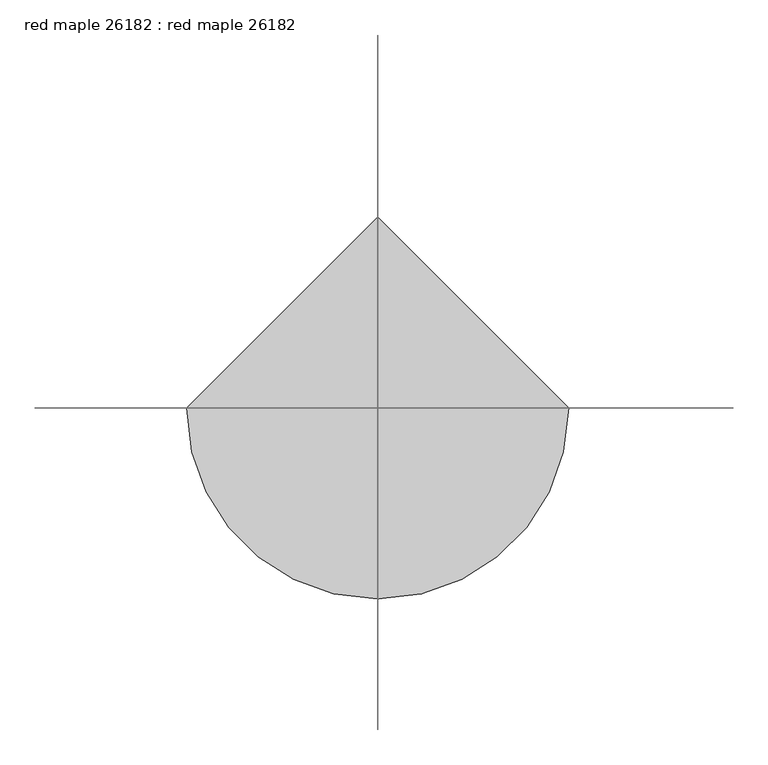
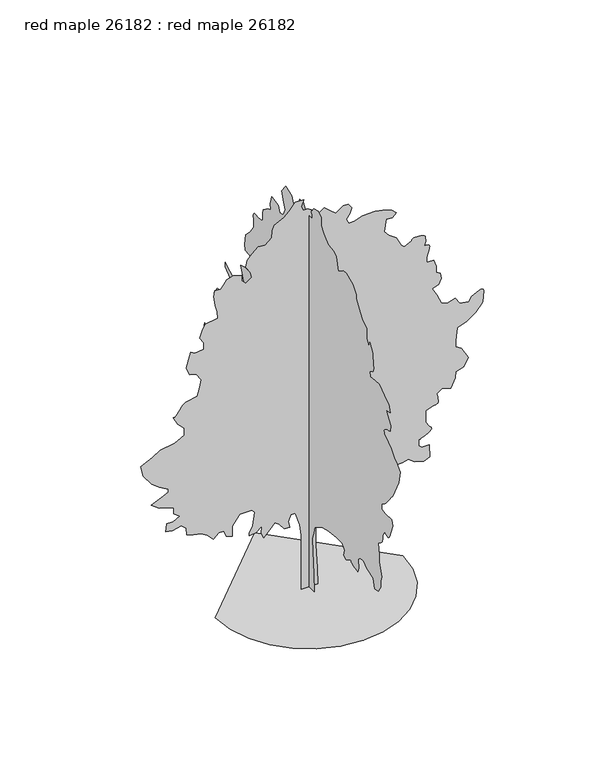
"""IFC4 building model written with IfcOpenShell, lengths in millimetres: proxy geometry, red maple 26182 : red maple 26182."""

import ifcopenshell
import ifcopenshell.guid

model = None  # the IFC model being written
_history = None  # IfcOwnerHistory: only IFC2X3 demands one
_inside = {}  # id of a spatial element -> (the spatial element, [elements in it])
_under = {}  # id of a project, library or spatial element -> (it, [spatial elements below it])
_declared = {}  # id of a project -> (the project, [libraries it declares])
_typed = {}  # id of a type object -> (the type object, [elements of that type])
_made_of = {}  # id of a material, layer set ... -> (it, [elements and type objects made of it])


def new_model(schema):
    """Start an empty IFC model of exactly this schema.

    Asked for "IFC4X3", IfcOpenShell would pick the latest addendum, in which some entities
    have other attributes; the version numbers below select the first issue.
    IFC2X3 requires an IfcOwnerHistory on every rooted entity: one is made here for all.
    """
    global model, _history
    if schema == "IFC4X3":
        model = ifcopenshell.file(schema_version=(4, 3, 0, 0))
    else:
        model = ifcopenshell.file(schema=schema)
    _inside.clear()
    _under.clear()
    _declared.clear()
    _typed.clear()
    _made_of.clear()
    _history = None
    if model.schema == "IFC2X3":
        org = make("IfcOrganization", Name="unknown")
        user = make(
            "IfcPersonAndOrganization",
            ThePerson=make("IfcPerson", FamilyName="unknown"),
            TheOrganization=org,
        )
        app = make(
            "IfcApplication",
            ApplicationDeveloper=org,
            Version="unknown",
            ApplicationFullName="unknown",
            ApplicationIdentifier="unknown",
        )
        _history = make(
            "IfcOwnerHistory",
            OwningUser=user,
            OwningApplication=app,
            ChangeAction="ADDED",
            CreationDate=0,
        )
    return model


def make(cls, **values):
    """One entity of the class cls with the attributes given. An attribute that is None is left unset."""
    return model.create_entity(
        cls, **{name: value for name, value in values.items() if value is not None}
    )


def rooted(cls, **values):
    """An entity with a GlobalId (a new one), such as an element, a storey or a relation."""
    return make(cls, GlobalId=ifcopenshell.guid.new(), OwnerHistory=_history, **values)


def si_unit(unit_type, name, prefix=None):
    """IfcSIUnit, for example si_unit("LENGTHUNIT", "METRE", prefix="MILLI")."""
    return make("IfcSIUnit", UnitType=unit_type, Prefix=prefix, Name=name)


def assignment(units):
    """IfcUnitAssignment: the units of a project."""
    return None if units is None else make("IfcUnitAssignment", Units=units)


def point(xyz):
    """IfcCartesianPoint."""
    return None if xyz is None else make("IfcCartesianPoint", Coordinates=xyz)


def direction(xyz):
    """IfcDirection."""
    return None if xyz is None else make("IfcDirection", DirectionRatios=xyz)


def frame(location, z_axis=None, x_axis=None):
    """IfcAxis2Placement3D, a coordinate frame: its origin and axes. An axis left out is left unset."""
    return make(
        "IfcAxis2Placement3D",
        Location=point(location),
        Axis=direction(z_axis),
        RefDirection=direction(x_axis),
    )


def origin():
    """The frame at (0, 0, 0) with its axes left unset."""
    return frame((0.0, 0.0, 0.0))


def place(relative_to, where):
    """IfcLocalPlacement: puts the frame where relative to a parent placement (None: the world)."""
    return make(
        "IfcLocalPlacement", PlacementRelTo=relative_to, RelativePlacement=where
    )


def context(
    kind, dimensions, precision=None, world=None, true_north=None, identifier=None
):
    """IfcGeometricRepresentationContext, for example the 3D "Model" context."""
    return make(
        "IfcGeometricRepresentationContext",
        ContextIdentifier=identifier,
        ContextType=kind,
        CoordinateSpaceDimension=dimensions,
        Precision=precision,
        WorldCoordinateSystem=world,
        TrueNorth=true_north,
    )


def project(units=None, contexts=None):
    """IfcProject with its units and contexts."""
    return rooted(
        "IfcProject",
        Name="project",
        RepresentationContexts=contexts,
        UnitsInContext=assignment(units),
    )


def spatial(cls, under=None, at=None, **own):
    """A site, building, storey or space (cls), placed at a placement, below another one or the project."""
    s = rooted(cls, ObjectPlacement=at, **own)
    if under is not None:
        _under.setdefault(under.id(), (under, []))[1].append(s)
    return s


def point_list(points):
    """IfcCartesianPointList2D or 3D."""
    cls = (
        "IfcCartesianPointList2D" if len(points[0]) == 2 else "IfcCartesianPointList3D"
    )
    return make(cls, CoordList=points)


def triangles(points, corners, closed=None, point_numbers=None):
    """IfcTriangulatedFaceSet: each triangle names its three corners, points numbered from 1."""
    return make(
        "IfcTriangulatedFaceSet",
        Coordinates=point_list(points),
        Closed=closed,
        CoordIndex=corners,
        PnIndex=point_numbers,
    )


def shape(context_of_items, identifier, shape_type, items):
    """IfcShapeRepresentation: the items that make up one representation, for example the "Body"."""
    return make(
        "IfcShapeRepresentation",
        ContextOfItems=context_of_items,
        RepresentationIdentifier=identifier,
        RepresentationType=shape_type,
        Items=items,
    )


def source(mapping_origin, context_of_items, identifier, shape_type, items):
    """IfcRepresentationMap: a shape defined once, which mapped items show again and again."""
    return make(
        "IfcRepresentationMap",
        MappingOrigin=mapping_origin,
        MappedRepresentation=shape(context_of_items, identifier, shape_type, items),
    )


def transform(
    local_origin,
    x_axis=None,
    y_axis=None,
    z_axis=None,
    scale=None,
    scale2=None,
    scale3=None,
    uniform=True,
):
    """IfcCartesianTransformationOperator3D, or its non-uniform kind. x_axis, y_axis, z_axis: its Axis1, 2, 3."""
    if uniform:
        return make(
            "IfcCartesianTransformationOperator3D",
            Axis1=direction(x_axis),
            Axis2=direction(y_axis),
            LocalOrigin=point(local_origin),
            Scale=scale,
            Axis3=direction(z_axis),
        )
    return make(
        "IfcCartesianTransformationOperator3DnonUniform",
        Axis1=direction(x_axis),
        Axis2=direction(y_axis),
        LocalOrigin=point(local_origin),
        Scale=scale,
        Axis3=direction(z_axis),
        Scale2=scale2,
        Scale3=scale3,
    )


def mapped(mapping_source, mapping_target):
    """IfcMappedItem: shows the shape of a source again, moved by a transform."""
    return make(
        "IfcMappedItem", MappingSource=mapping_source, MappingTarget=mapping_target
    )


def made_of(thing, what):
    """Note that an element or type object is made of a material, layer set ...; save() writes the relation."""
    if what is not None:
        _made_of.setdefault(what.id(), (what, []))[1].append(thing)
    return thing


def element(
    cls,
    number,
    at=None,
    inside=None,
    cuts=None,
    type_object=None,
    material=None,
    context=None,
    identifier="Body",
    shape_type=None,
    held_by="IfcProductDefinitionShape",
    body=None,
    shapes=None,
    **own,
):
    """One element of the class cls, such as IfcWall. Its Tag is "e" and its number.

    at: its placement. inside: the storey or other place that contains it. cuts: it is an
    opening in that element (IfcRelVoidsElement). A single representation is given by context,
    identifier, shape_type and body (its items); several are given by shapes. held_by: the class
    of the entity that holds the representations. save() writes the other relations.
    """
    e = rooted(cls, Tag="e%d" % number, ObjectPlacement=at, **own)
    if body is not None:
        shapes = [shape(context, identifier, shape_type, body)]
    if shapes is not None:
        e.Representation = make(held_by, Representations=shapes)
    if inside is not None:
        _inside.setdefault(inside.id(), (inside, []))[1].append(e)
    if cuts is not None:
        rooted(
            "IfcRelVoidsElement", RelatingBuildingElement=cuts, RelatedOpeningElement=e
        )
    if type_object is not None:
        _typed.setdefault(type_object.id(), (type_object, []))[1].append(e)
    return made_of(e, material)


def aggregate(whole, parts):
    """IfcRelAggregates: a whole, such as a stair, and the parts it consists of."""
    return rooted("IfcRelAggregates", RelatingObject=whole, RelatedObjects=parts)


def save(model, path):
    """Write the relations noted so far, then the file.

    IfcRelAggregates (storeys below a building ...), IfcRelContainedInSpatialStructure (elements
    in a storey), IfcRelDefinesByType, IfcRelAssociatesMaterial and IfcRelDeclares: one each for
    every whole, place, type object, material and project.
    """
    for whole, parts in _under.values():
        aggregate(whole, parts)
    for where, things in _inside.values():
        rooted(
            "IfcRelContainedInSpatialStructure",
            RelatedElements=things,
            RelatingStructure=where,
        )
    for kind, things in _typed.values():
        rooted("IfcRelDefinesByType", RelatedObjects=things, RelatingType=kind)
    for what, things in _made_of.values():
        rooted("IfcRelAssociatesMaterial", RelatedObjects=things, RelatingMaterial=what)
    for by, libraries in _declared.values():
        rooted("IfcRelDeclares", RelatingContext=by, RelatedDefinitions=libraries)
    model.write(path)


def red_maple_26182_red_maple_26182_cba750cc(model_context):
    return source(origin(), model_context, "Body", "Tessellation", [
        triangles([(5.9e-06, 200.5240248, 0.0131599), (5.9e-06, -200.5423013, 0.0131599), (5.9e-06, -173.8047255, 401.079007), (5.9e-06, -147.0663684, 922.4677488), (5.9e-06, -133.6980892, 1216.5822092), (5.9e-06, -173.8047255, 1363.6407475), (5.9e-06, -227.2806583, 1537.4352264), (5.9e-06, -320.8632274, 1590.9124855), (5.9e-06, -534.7644153, 1711.2323215), (5.9e-06, -762.0361897, 1764.7071098), (5.9e-06, -1069.5212002, 1804.8136734), (5.9e-06, -1283.4223881, 1804.8136734), (5.9e-06, -1377.0037399, 1697.8617714), (5.9e-06, -1336.897031, 1550.8033058), (5.9e-06, -1443.848933, 1510.6967422), (5.9e-06, -1617.6460281, 1604.2805649), (5.9e-06, -1620.762553, 1592.8200726), (5.9e-06, -1625.400642, 1581.362051), (5.9e-06, -1633.0790977, 1569.9041748), (5.9e-06, -1645.319339, 1558.4436825), (5.9e-06, -1663.6378429, 1546.9856609), (5.9e-06, -1689.5560284, 1535.5251686), (5.9e-06, -1724.595314, 1524.0672924), (5.9e-06, -1761.1942429, 1514.1662979), (5.9e-06, -1791.4812023, 1507.0721088), (5.9e-06, -1816.5027855, 1502.3197826), (5.9e-06, -1837.3156139, 1499.4343483), (5.9e-06, -1854.971077, 1497.9534794), (5.9e-06, -1870.5234707, 1497.4074371), (5.9e-06, -1885.021859, 1497.3286629), (5.9e-06, -1911.7604885, 1590.9124855), (5.9e-06, -1898.3924091, 1791.445594), (5.9e-06, -1978.6056816, 1871.6588665), (5.9e-06, -2112.293597, 1885.0269459), (5.9e-06, -2219.245499, 1778.0750439), (5.9e-06, -2473.2533958, 1697.8617714), (5.9e-06, -2540.1036758, 1497.3286629), (5.9e-06, -2660.4236572, 1510.6967422), (5.9e-06, -2767.3575371, 1671.125758), (5.9e-06, -2767.3575371, 1804.8136734), (5.9e-06, -2794.1038696, 1911.7655754), (5.9e-06, -2700.5302208, 2219.2479698), (5.9e-06, -2700.5302208, 2393.0450649), (5.9e-06, -2673.7838882, 2660.4236572), (5.9e-06, -2676.8572472, 2660.5759735), (5.9e-06, -2681.2261665, 2661.668058), (5.9e-06, -2688.1603363, 2664.6399696), (5.9e-06, -2698.9553169, 2670.4056061), (5.9e-06, -2714.9066689, 2679.9053169), (5.9e-06, -2737.284082, 2694.1038689), (5.9e-06, -2767.3575371, 2713.8904518), (5.9e-06, -2796.66912, 2738.3761665), (5.9e-06, -2816.8623642, 2765.6558968), (5.9e-06, -2829.4607231, 2795.2721123), (5.9e-06, -2835.9629425, 2826.7681549), (5.9e-06, -2837.9189278, 2859.6612053), (5.9e-06, -2836.8265526, 2893.4940239), (5.9e-06, -2834.2104332, 2927.8096619), (5.9e-06, -2914.423851, 3061.4898743), (5.9e-06, -2945.8434448, 3041.8556076), (5.9e-06, -2976.6790627, 3024.6598549), (5.9e-06, -3006.3211487, 3012.3917084), (5.9e-06, -3034.2357239, 3007.4641022), (5.9e-06, -3059.8135231, 3012.3917084), (5.9e-06, -3082.4449905, 3029.5618813), (5.9e-06, -3101.5964378, 3061.4898743), (5.9e-06, -3235.2766502, 3382.3429642), (5.9e-06, -3195.1700867, 3516.0231766), (5.9e-06, -2941.1698929, 3502.6629456), (5.9e-06, -2794.1038696, 3516.0231766), (5.9e-06, -2807.4641006, 3649.7289688), (5.9e-06, -2841.8811859, 3670.0236603), (5.9e-06, -2876.5523254, 3691.8420959), (5.9e-06, -2911.6551247, 3716.7088921), (5.9e-06, -2947.4692177, 3746.1475021), (5.9e-06, -2984.2230789, 3781.6566719), (5.9e-06, -3022.1707626, 3824.7604362), (5.9e-06, -3061.4898743, 3876.98283), (5.9e-06, -3098.0914192, 3928.4433517), (5.9e-06, -3128.3680595, 3969.3626564), (5.9e-06, -3153.3871719, 4001.5191238), (5.9e-06, -3174.2152611, 4026.6652634), (5.9e-06, -3191.8682533, 4046.5280045), (5.9e-06, -3207.412944, 4062.9110161), (5.9e-06, -3221.9164192, 4077.5159386), (5.9e-06, -3449.1958603, 4532.0748207), (5.9e-06, -3516.0231766, 4826.1815781), (5.9e-06, -3368.9824425, 4986.6084137), (5.9e-06, -3302.1295464, 4999.9686447), (5.9e-06, -3155.0635231, 5187.1415222), (5.9e-06, -3061.4898743, 5253.9944183), (5.9e-06, -3024.5075386, 5271.2916183), (5.9e-06, -2989.023658, 5289.3004028), (5.9e-06, -2956.5878471, 5308.7056137), (5.9e-06, -2928.7238503, 5330.2194168), (5.9e-06, -2906.9559929, 5354.5528152), (5.9e-06, -2892.7574409, 5382.3656525), (5.9e-06, -2887.6775185, 5414.4206726), (5.9e-06, -2894.7134262, 5445.6629517), (5.9e-06, -2914.3474022, 5471.3166183), (5.9e-06, -2944.5228859, 5492.2973145), (5.9e-06, -2983.1054146, 5509.5183563), (5.9e-06, -3028.0125572, 5523.9453827), (5.9e-06, -3077.1107231, 5536.493454), (5.9e-06, -3128.3171906, 5548.100885), (5.9e-06, -3141.7030014, 5695.1669083), (5.9e-06, -3074.850396, 5802.1010788), (5.9e-06, -2967.8906456, 5949.1671021), (5.9e-06, -3128.3171906, 5989.2739563), (5.9e-06, -3074.850396, 6149.7007919), (5.9e-06, -2901.0633293, 6256.6599609), (5.9e-06, -2700.5302208, 6403.7009857), (5.9e-06, -2526.7306549, 6390.3401733), (5.9e-06, -2366.3039646, 6376.9799423), (5.9e-06, -2339.5653351, 6483.9141129), (5.9e-06, -2419.7786076, 6537.4061966), (5.9e-06, -2434.0052101, 6540.4798462), (5.9e-06, -2447.6476913, 6544.8487656), (5.9e-06, -2460.1190231, 6551.7826447), (5.9e-06, -2470.8378456, 6562.577916), (5.9e-06, -2479.217276, 6578.5292679), (5.9e-06, -2484.6730476, 6600.9063904), (5.9e-06, -2486.6238007, 6630.9801361), (5.9e-06, -2485.4529419, 6668.4702896), (5.9e-06, -2482.1813393, 6711.5746353), (5.9e-06, -2477.1522858, 6759.3769501), (5.9e-06, -2470.7209923, 6810.8883408), (5.9e-06, -2463.2380188, 6865.2193268), (5.9e-06, -2455.0515999, 6921.4292679), (5.9e-06, -2446.5172371, 6978.5792679), (5.9e-06, -2339.5653351, 7165.7521454), (5.9e-06, -2299.4587715, 7058.792395), (5.9e-06, -2232.6135784, 7179.1123764), (5.9e-06, -2232.6135784, 7433.1125702), (5.9e-06, -2058.8189541, 7540.0723206), (5.9e-06, -1938.499118, 7700.4985748), (5.9e-06, -1818.1791367, 7874.2856415), (5.9e-06, -1818.1791367, 7967.8845795), (5.9e-06, -1684.4887505, 8128.3114151), (5.9e-06, -1443.848933, 8248.6313965), (5.9e-06, -1310.1610176, 8221.8847733), (5.9e-06, -1136.3639225, 8101.5647919), (5.9e-06, -1042.7825706, 8395.6718399), (5.9e-06, -949.198748, 8462.524736), (5.9e-06, -735.2975601, 8489.2707779), (5.9e-06, -574.8710515, 8649.6976135), (5.9e-06, -467.9217293, 8770.0175949), (5.9e-06, -467.9217293, 8957.1648926), (5.9e-06, -347.6018206, 9037.3780197), (5.9e-06, -187.1730047, 8997.2711655), (5.9e-06, -93.5917073, 8876.9517654), (5.9e-06, -107.5840764, 8845.6589081), (5.9e-06, -119.5886307, 8815.6357407), (5.9e-06, -127.6175737, 8788.2036942), (5.9e-06, -129.6833633, 8764.6324585), (5.9e-06, -123.7979213, 8746.192305), (5.9e-06, -107.9734512, 8734.1779221), (5.9e-06, -80.2224107, 8729.9107407), (5.9e-06, 106.9427183, 8729.9107407), (5.9e-06, 227.262618, 8903.6978073), (5.9e-06, 360.9520595, 8890.3375763), (5.9e-06, 427.7947454, 8729.9107407), (5.9e-06, 601.5918769, 8649.6976135), (5.9e-06, 668.4345629, 8783.3778259), (5.9e-06, 895.7063009, 8876.9517654), (5.9e-06, 1042.7648392, 8676.4180756), (5.9e-06, 975.9195734, 8449.164505), (5.9e-06, 922.4449305, 8302.0984818), (5.9e-06, 989.2901236, 8141.6716461), (5.9e-06, 1122.9781116, 8114.9256042), (5.9e-06, 1176.4527546, 8261.9916275), (5.9e-06, 1443.8312016, 8288.7376694), (5.9e-06, 1497.3083153, 8101.5647919), (5.9e-06, 1470.5696857, 7967.8845795), (5.9e-06, 1590.8896671, 7927.7783066), (5.9e-06, 1764.6841461, 7794.0725143), (5.9e-06, 1778.0546963, 7700.4985748), (5.9e-06, 1778.0546963, 7540.0723206), (5.9e-06, 1844.8974186, 7499.9654663), (5.9e-06, 2005.3239635, 7499.9654663), (5.9e-06, 2036.5838287, 7505.2994431), (5.9e-06, 2066.3221298, 7508.2969345), (5.9e-06, 2093.0200642, 7506.6202927), (5.9e-06, 2115.1586838, 7497.9336136), (5.9e-06, 2131.2167152, 7479.8998306), (5.9e-06, 2139.6749199, 7450.1562973), (5.9e-06, 2139.0144951, 7406.3921082), (5.9e-06, 2134.0639252, 7358.3095779), (5.9e-06, 2130.5182114, 7316.5772415), (5.9e-06, 2128.1407402, 7280.1033051), (5.9e-06, 2126.6979504, 7247.8198105), (5.9e-06, 2125.9562805, 7218.7111221), (5.9e-06, 2125.6844948, 7191.6854462), (5.9e-06, 2125.6464157, 7165.7521454), (5.9e-06, 2259.3343311, 6978.5792679), (5.9e-06, 2433.1289555, 6804.7922012), (5.9e-06, 2473.2356644, 6550.767009), (5.9e-06, 2446.4995056, 6430.4470276), (5.9e-06, 2312.8089741, 6417.0867966), (5.9e-06, 2205.8596882, 6390.3401733), (5.9e-06, 2125.6464157, 6216.5531067), (5.9e-06, 2232.5957016, 6016.0199982), (5.9e-06, 2473.2356644, 6016.0199982), (5.9e-06, 2633.6520355, 5962.5279144), (5.9e-06, 2499.9741486, 5614.9537811), (5.9e-06, 2620.2915138, 5481.2479889), (5.9e-06, 2954.5048347, 5521.3548431), (5.9e-06, 3048.1040634, 5574.8475082), (5.9e-06, 3235.2513611, 5668.4208664), (5.9e-06, 3221.8908394, 5574.8475082), (5.9e-06, 2981.2511673, 5360.9280075), (5.9e-06, 2887.6775185, 5066.8215408), (5.9e-06, 2994.611689, 4839.5420998), (5.9e-06, 3141.6777122, 4852.9279106), (5.9e-06, 3144.9033875, 4867.1011734), (5.9e-06, 3150.3643913, 4880.4869843), (5.9e-06, 3160.2704727, 4892.2217331), (5.9e-06, 3176.8313805, 4901.4926788), (5.9e-06, 3202.2821526, 4907.4870804), (5.9e-06, 3238.8581177, 4909.3921967), (5.9e-06, 3288.7437355, 4906.3947052), (5.9e-06, 3529.3836983, 4879.6486633), (5.9e-06, 3649.703389, 4705.8618874), (5.9e-06, 3609.5968254, 4518.6890099), (5.9e-06, 3462.5308022, 4411.7548393), (5.9e-06, 3342.2108208, 4117.6227928), (5.9e-06, 3395.677906, 3930.4752045), (5.9e-06, 3449.1702805, 3863.622599), (5.9e-06, 3582.8507835, 3636.343158), (5.9e-06, 3850.2367882, 3663.0891998), (5.9e-06, 4024.0235641, 3770.0489502), (5.9e-06, 4077.4906494, 3529.4089874), (5.9e-06, 3823.4904556, 3409.089006), (5.9e-06, 3649.703389, 3355.5966316), (5.9e-06, 3529.3836983, 3088.2362068), (5.9e-06, 3462.5308022, 2927.8096619), (5.9e-06, 3382.3173843, 2700.5302208), (5.9e-06, 3235.2513611, 2727.2762627), (5.9e-06, 3007.9974998, 2767.3831169), (5.9e-06, 2820.8246223, 2727.2762627), (5.9e-06, 2687.1444099, 2513.364901), (5.9e-06, 2860.9311859, 2339.570422), (5.9e-06, 3021.3577309, 2312.8319378), (5.9e-06, 3048.1040634, 2058.8215702), (5.9e-06, 3036.4454727, 2033.2918785), (5.9e-06, 3023.6183487, 2009.2838963), (5.9e-06, 3008.4547394, 1988.3135193), (5.9e-06, 2989.7855301, 1971.9052185), (5.9e-06, 2966.4430595, 1961.5775059), (5.9e-06, 2937.258213, 1958.8496201), (5.9e-06, 2901.0380402, 1965.2402184), (5.9e-06, 2863.2679619, 1977.8690987), (5.9e-06, 2829.7147774, 1992.6010483), (5.9e-06, 2799.6663208, 2009.0882687), (5.9e-06, 2772.4121704, 2026.9800545), (5.9e-06, 2747.2916107, 2045.9209042), (5.9e-06, 2723.5424789, 2065.5651993), (5.9e-06, 2700.504641, 2085.5600544), (5.9e-06, 2606.9309921, 2192.5119564), (5.9e-06, 2589.5829231, 2220.7695339), (5.9e-06, 2571.2947952, 2246.6877193), (5.9e-06, 2551.1527107, 2267.9297367), (5.9e-06, 2528.193647, 2282.1561939), (5.9e-06, 2501.4929512, 2287.0279896), (5.9e-06, 2470.1189941, 2280.208057), (5.9e-06, 2433.1289555, 2259.3571495), (5.9e-06, 2386.7865807, 2232.2681053), (5.9e-06, 2329.2174202, 2207.9857212), (5.9e-06, 2262.2959236, 2186.0425838), (5.9e-06, 2187.8891281, 2165.9689545), (5.9e-06, 2107.8714832, 2147.2998905), (5.9e-06, 2024.1123516, 2129.5656532), (5.9e-06, 1938.4812412, 2112.2986839), (5.9e-06, 1724.5775826, 2058.8215702), (5.9e-06, 1791.4227757, 1925.1335094), (5.9e-06, 2005.3239635, 1791.445594), (5.9e-06, 2112.2758656, 1617.6484989), (5.9e-06, 1925.1106911, 1550.8033058), (5.9e-06, 1899.2305847, 1550.9989334), (5.9e-06, 1872.766357, 1552.362949), (5.9e-06, 1845.1311253, 1556.0662113), (5.9e-06, 1815.7433842, 1563.2772537), (5.9e-06, 1784.0161057, 1575.1644642), (5.9e-06, 1749.3654591, 1592.8988468), (5.9e-06, 1711.2095032, 1617.6484989), (5.9e-06, 1671.8826885, 1646.6858253), (5.9e-06, 1633.9579685, 1676.4242718), (5.9e-06, 1597.2041073, 1706.7493103), (5.9e-06, 1561.3849274, 1737.539146), (5.9e-06, 1526.2668674, 1768.6821579), (5.9e-06, 1491.6162209, 1800.0587311), (5.9e-06, 1457.1991356, 1831.5523029), (5.9e-06, 1189.8233047, 1911.7655754), (5.9e-06, 975.9195734, 1951.872139), (5.9e-06, 762.0183855, 2005.3467819), (5.9e-06, 548.1146542, 1965.2402184), (5.9e-06, 253.9999576, 1858.2883163), (5.9e-06, 173.7866851, 1751.3390305), (5.9e-06, 106.9427183, 1564.173856), (5.9e-06, 80.2041161, 1296.7955544), (5.9e-06, 106.9427183, 935.8358282), (5.9e-06, 160.4173885, 414.4495934), (-2085.2019367, 0.0, 0.0), (-2030.0762318, -477.7896226, 0.0), (-1873.078838, -916.5648388, 0.0), (-1626.7799183, -1303.7500717, 0.0), (-1303.7500717, -1626.7799183, 0.0), (-916.5648388, -1873.078838, 0.0), (-477.7896226, -2030.0762318, 0.0), (9.11e-05, -2085.2019367, 0.0), (477.7896226, -2030.0762318, 0.0), (916.5648388, -1873.078838, 0.0), (1303.7500717, -1626.7799183, 0.0), (1626.7799183, -1303.7500717, 0.0), (1873.078838, -916.5648388, 0.0), (2030.0762318, -477.7896226, 0.0), (2085.2019367, 0.0001828, 0.0), (-0.0002734, 2085.2019367, 0.0), (199.8874902, 0.0002285, 0.005264), (-169.704903, 0.0002285, 0.005264), (-169.704903, 0.0001919, 684.4365658), (-169.704903, 0.0001645, 1040.3416586), (-169.704903, 0.0001554, 1273.0464226), (-210.770892, 0.0001371, 1533.1325821), (-306.5909517, 0.0001188, 1834.2801888), (-402.4125375, 0.0001188, 1834.2801888), (-457.1673348, 0.0001279, 1683.7063854), (-429.7886644, 0.0001371, 1546.8205547), (-552.9863771, 0.0001371, 1560.5086727), (-662.4960445, 0.0001279, 1697.3945034), (-758.317594, 0.0001279, 1765.8374187), (-867.8247179, 0.0001279, 1642.639706), (-1004.7104759, 0.0001371, 1505.7538754), (-1059.465346, 0.0001371, 1628.9515881), (-1045.777228, 0.0001279, 1793.2159801), (-1182.6630587, 0.0001279, 1683.7063854), (-1333.2394054, 0.0001279, 1670.0182674), (-1333.2394054, 0.0001279, 1738.4611828), (-1251.1059013, 0.0001188, 1875.3470135), (-1210.0416927, 0.0001005, 2176.4972363), (-1278.4846081, 0.0001005, 2244.9401516), (-1538.5681515, 0.0001005, 2244.9401516), (-1702.8300728, 0.0001097, 2012.2328442), (-1702.8300728, 0.0001188, 1916.4136929), (-1702.8300728, 0.0001279, 1779.5280075), (-1839.7183743, 0.0001188, 1834.2801888), (-1894.4731716, 0.0001097, 1971.1686356), (-2003.9802956, 0.0001097, 1971.1686356), (-2127.1780083, 0.0001188, 1861.6588955), (-2264.063839, 0.0001097, 1998.5447262), (-2400.9521404, 0.0001097, 2080.6756142), (-2578.9149696, 0.0001005, 2121.7424389), (-2715.7955681, 0.0001005, 2176.4972363), (-2729.4863022, 9.14e-05, 2327.0711849), (-2838.9857231, 8.22e-05, 2422.8926617), (-3044.3194107, 9.14e-05, 2381.8259823), (-3181.2000092, 8.22e-05, 2409.204689), (-3167.5095657, 7.31e-05, 2587.1444092), (-3016.9382332, 7.31e-05, 2587.1444092), (-2880.0576347, 7.31e-05, 2669.2882324), (-3003.2474991, 6.4e-05, 2765.0969193), (-3003.2474991, 5.48e-05, 2902.0030975), (-3140.1283882, 5.48e-05, 2956.7401634), (-3331.7713417, 5.48e-05, 3011.5025185), (-3509.7241425, 4.57e-05, 3148.3834076), (-3290.6997208, 3.66e-05, 3244.2176743), (-3126.4376541, 3.66e-05, 3312.6451836), (-3126.4376541, 2.74e-05, 3381.0982727), (-3331.7713417, 1.83e-05, 3504.2884277), (-3496.0334084, 1.83e-05, 3627.5038719), (-3687.6766525, 0.0, 3887.5746254), (-3742.4390076, -1.83e-05, 4133.9802246), (-3632.9395866, -1.83e-05, 4188.7172905), (-3482.3426743, -2.74e-05, 4257.1703796), (-3304.3901642, -2.74e-05, 4366.6698006), (-2989.5570557, -3.66e-05, 4421.4324463), (-2770.532634, -3.66e-05, 4530.9318672), (-2770.532634, -4.57e-05, 4695.1936432), (-2921.1292557, -5.48e-05, 4845.7905556), (-3016.9382332, -7.31e-05, 5023.742775), (-3007.9974998, -7.31e-05, 5021.1266556), (-2998.2184456, -7.31e-05, 5020.5679688), (-2986.7630402, -7.31e-05, 5024.0985672), (-2972.7929626, -7.31e-05, 5033.6997253), (-2955.4701828, -7.31e-05, 5051.4544556), (-2933.9816689, -7.31e-05, 5079.3946106), (-2907.4388123, -7.31e-05, 5119.5520432), (-2879.295472, -7.31e-05, 5162.0971207), (-2853.3113022, -8.22e-05, 5196.7426804), (-2829.1305107, -8.22e-05, 5224.783992), (-2806.3720161, -8.22e-05, 5247.5680664), (-2784.7058968, -8.22e-05, 5266.4145905), (-2763.7507805, -8.22e-05, 5282.6199966), (-2743.1767456, -8.22e-05, 5297.5045532), (-2483.0830284, -9.14e-05, 5352.2669083), (-2428.328231, -0.0001005, 5543.9098618), (-2400.9521404, -0.0001097, 5708.1719284), (-2510.4618805, -0.0001188, 5872.4339951), (-2647.3424789, -0.0001188, 5913.4803268), (-2729.4863022, -0.0001371, 6091.4328369), (-2674.7236565, -0.0001462, 6283.0757904), (-2633.6520355, -0.0001554, 6433.6474136), (-2537.8378258, -0.0001462, 6378.9100571), (-2346.1973431, -0.0001554, 6406.2915253), (-2346.1973431, -0.0001645, 6556.8625671), (-2428.328231, -0.0001645, 6693.7437469), (-2373.5734337, -0.0001736, 6844.3147888), (-2305.1305183, -0.0001828, 6981.1953873), (-2031.3590023, -0.0001919, 7022.2672989), (-2045.0471203, -0.0002011, 7186.5293655), (-2086.1137997, -0.0002102, 7337.1004074), (-2113.4900356, -0.0002193, 7556.1248291), (-2099.8019176, -0.0002285, 7693.0060089), (-1962.916087, -0.0002285, 7679.3149841), (-1894.4731716, -0.0002285, 7761.4588074), (-1826.0302563, -0.0002376, 7857.2674942), (-1689.1419548, -0.0002376, 7898.3394058), (-1497.5013268, -0.0002376, 7843.5770508), (-1497.5013268, -0.0002285, 7720.3868958), (-1401.6823208, -0.0002285, 7624.5782089), (-1278.4846081, -0.0002285, 7720.3868958), (-1305.8606987, -0.0002376, 7857.2674942), (-1401.6823208, -0.0002467, 8007.8391174), (-1374.303614, -0.0002559, 8158.4357391), (-1264.7940193, -0.000265, 8267.9354507), (-1127.9081886, -0.0002742, 8391.1250244), (-977.3343853, -0.000265, 8377.434581), (-826.7605093, -0.0002742, 8500.6503159), (-813.0699205, -0.0002833, 8651.2213577), (-772.0057119, -0.0002924, 8774.4115128), (-566.6744588, -0.0003016, 8870.2457794), (-443.4767461, -0.0003016, 8979.745491), (-306.5909517, -0.0003107, 9144.0075577), (-114.9505871, -0.0003107, 9144.0075577), (-169.704903, -0.0003016, 8993.4359344), (-128.6391684, -0.0003016, 8897.6016678), (-32.8188589, -0.0003016, 8897.6016678), (49.3128694, -0.0002924, 8842.8648926), (76.6900319, -0.0002924, 8733.3396011), (240.9532249, -0.0002924, 8719.6491577), (336.7737751, -0.0002924, 8788.1019562), (473.6595695, -0.0002833, 8678.6028259), (596.8572822, -0.0002833, 8569.0781158), (761.1217833, -0.0002833, 8692.2932693), (870.6314507, -0.0002833, 8692.2932693), (952.7624113, -0.0002833, 8582.7685593), (911.6956593, -0.0002742, 8445.8879608), (829.5646986, -0.000265, 8350.0786926), (884.319496, -0.000265, 8240.5539825), (1007.5172087, -0.000265, 8240.5539825), (1199.1578367, -0.000265, 8309.006781), (1472.9294254, -0.000265, 8309.006781), (1637.1938175, -0.000265, 8281.6258942), (1842.5225636, -0.0002559, 8213.1725143), (1938.3441856, -0.0002559, 8117.3638275), (1856.2106815, -0.0002467, 8021.5295609), (1719.3248508, -0.0002467, 8035.2200043), (1691.9487602, -0.0002376, 7912.0298492), (1678.2580261, -0.0002285, 7761.4588074), (1774.0796482, -0.0002285, 7638.2686523), (1938.3441856, -0.0002193, 7528.7439423), (2047.8513096, -0.0002011, 7309.7195206), (2116.2940796, -0.0002011, 7254.982164), (2280.558617, -0.0002102, 7337.1004074), (2283.7919952, -0.0002102, 7348.7589981), (2288.8187233, -0.0002102, 7359.9350601), (2297.439418, -0.0002102, 7370.1460648), (2311.4475746, -0.0002102, 7378.9344818), (2332.6388683, -0.0002102, 7385.7927841), (2362.8089745, -0.0002102, 7390.2628601), (2403.7563297, -0.0002102, 7391.8633438), (2446.2989365, -0.0002102, 7390.2628601), (2480.9392639, -0.0002102, 7385.7927841), (2508.9962723, -0.0002102, 7378.9344818), (2531.7826721, -0.0002102, 7370.1460648), (2550.619313, -0.0002102, 7359.9350601), (2566.8244286, -0.0002102, 7348.7589981), (2581.7089851, -0.0002102, 7337.1004074), (2595.3994286, -0.0002011, 7213.9108337), (2568.018251, -0.0001919, 7118.1015656), (2599.8953751, -0.0001919, 7117.6446167), (2629.5115906, -0.0001919, 7114.5709671), (2654.581572, -0.0001919, 7106.2400803), (2672.8188309, -0.0001919, 7089.9840958), (2681.9627495, -0.0001919, 7063.2124741), (2679.7274208, -0.0001919, 7023.2579361), (2663.8525177, -0.0001828, 6967.5049438), (2643.9641968, -0.0001828, 6908.5771454), (2630.5530968, -0.0001828, 6859.6818741), (2622.5268425, -0.0001736, 6819.1686493), (2618.8183479, -0.0001736, 6785.3614105), (2618.3358192, -0.0001736, 6756.6085144), (2620.0121704, -0.0001736, 6731.1833221), (2622.7806061, -0.0001736, 6707.4341904), (2773.3519386, -0.0001736, 6707.4341904), (2828.1145844, -0.0001554, 6543.1721237), (2828.1145844, -0.0001554, 6406.2915253), (2923.9232712, -0.0001462, 6351.5291702), (2937.6140053, -0.0001371, 6228.3390152), (2882.8516502, -0.0001371, 6105.1232803), (2745.9707611, -0.0001279, 6050.3865051), (2841.8050278, -0.0001188, 5872.4339951), (2937.6140053, -0.0001097, 5653.4095734), (3074.4946037, -0.0001005, 5584.9561935), (3252.4471138, -0.0001097, 5639.7191299), (3348.2813805, -0.0001005, 5489.1475067), (3553.5897789, -9.14e-05, 5461.7666199), (3622.042868, -0.0001005, 5557.5753067), (3677.3894897, -0.0001005, 5589.3251129), (3730.4754936, -0.0001005, 5617.7989563), (3779.0149727, -0.0001097, 5639.8458664), (3820.6964401, -0.0001097, 5652.1648819), (3853.3101471, -0.0001097, 5651.5806152), (3874.5446068, -0.0001097, 5634.8165222), (3882.1392014, -0.0001005, 5598.6472183), (3881.3261696, -0.0001005, 5553.3081253), (3879.0911316, -0.0001005, 5510.8647858), (3875.6619804, -9.14e-05, 5470.7835114), (3871.2677719, -9.14e-05, 5432.6323517), (3866.1625603, -9.14e-05, 5395.9293594), (3860.5745293, -9.14e-05, 5360.1664261), (3854.7580238, -9.14e-05, 5324.8854401), (3704.1866913, -7.31e-05, 5160.6239548), (3512.5434471, -6.4e-05, 5010.0523315), (3293.5190254, -6.4e-05, 4941.5995331), (3266.1378479, -4.57e-05, 4640.4565773), (3266.1378479, -3.66e-05, 4503.5506897), (3389.3280029, -3.66e-05, 4421.4324463), (3539.9246246, -1.83e-05, 4161.336113), (3444.090358, -9.1e-06, 3969.7184486), (3266.1378479, 0.0, 3914.9558029), (3252.4471138, 9.1e-06, 3778.0752045), (3156.638427, 1.83e-05, 3559.0507828), (2964.9951828, 1.83e-05, 3627.5038719), (2846.3771324, 1.83e-05, 3536.8765549), (2845.4879425, 1.83e-05, 3538.3244316), (2845.1071518, 1.83e-05, 3537.5369797), (2845.7675766, 1.83e-05, 3532.3047409), (2847.9773254, 1.83e-05, 3520.3665161), (2852.269796, 1.83e-05, 3499.5131378), (2859.1786766, 2.74e-05, 3467.5345665), (2869.1609161, 2.74e-05, 3422.1701843), (2875.307634, 2.74e-05, 3376.1453773), (2871.3959541, 2.74e-05, 3342.3378479), (2859.1025185, 3.66e-05, 3318.7157433), (2840.1286766, 3.66e-05, 3303.2219215), (2816.1002014, 3.66e-05, 3293.8492378), (2788.7190239, 3.66e-05, 3288.5405502), (2759.6614952, 3.66e-05, 3285.264006), (2595.3994286, 3.66e-05, 3230.5269402), (2595.3994286, 5.48e-05, 2956.7401634), (2677.517672, 6.4e-05, 2833.5500084), (2697.53302, 6.4e-05, 2815.871727), (2714.297113, 6.4e-05, 2797.7106262), (2724.5839851, 6.4e-05, 2778.5844681), (2725.1682518, 6.4e-05, 2758.0357224), (2712.8492363, 6.4e-05, 2735.582151), (2684.3503944, 7.31e-05, 2710.7156456), (2636.4713402, 7.31e-05, 2682.9786758), (2584.1727882, 7.31e-05, 2657.2229805), (2543.4055092, 7.31e-05, 2637.9697952), (2512.1864845, 7.31e-05, 2624.0761665), (2488.640538, 7.31e-05, 2614.5002975), (2470.8427872, 7.31e-05, 2608.1503944), (2456.8753258, 7.31e-05, 2603.9593712), (2444.8231544, 7.31e-05, 2600.8351433), (2444.8231544, 8.22e-05, 2463.9594864), (2513.2660698, 9.14e-05, 2395.5139549), (2677.517672, 9.14e-05, 2395.5139549), (2691.2084061, 0.0001005, 2108.0543209), (2554.3275169, 0.0001097, 2053.2995235), (2349.0015324, 0.0001005, 2121.7424389), (2212.1157017, 0.0001005, 2217.564061), (2075.229871, 0.0001005, 2190.1853542), (1828.8344456, 0.0001005, 2176.4972363), (1678.2580261, 0.0001005, 2135.4305569), (1664.5700535, 0.0001188, 1943.7899288), (1513.9961048, 0.0001188, 1930.1018108), (1322.3554768, 0.0001188, 1943.7899288), (1240.2219727, 0.0001188, 1820.5922161), (952.7624113, 0.0001279, 1779.5280075), (733.7430765, 0.0001188, 1834.2801888), (733.7430765, 0.0001371, 1615.2634701), (555.7930736, 0.0001371, 1628.9515881), (501.0382762, 0.0001279, 1738.4611828), (405.2166904, 0.0001279, 1697.3945034), (295.7070412, 0.0001279, 1697.3945034), (254.6428326, 0.0001188, 1820.5922161), (145.13292, 0.0001279, 1697.3945034), (131.4443387, 0.0001371, 1546.8205547), (145.13292, 0.0001554, 1314.1132473), (145.13292, 0.0001736, 930.8319912), (186.1989181, 0.0002102, 383.2863067)], [[130, 131, 132], [208, 209, 210], [208, 210, 211], [207, 208, 211], [230, 231, 232], [230, 232, 233], [276, 277, 278], [229, 230, 233], [229, 233, 234], [302, 1, 2], [302, 2, 3], [302, 3, 4], [301, 302, 4], [301, 4, 5], [300, 301, 5], [300, 5, 6], [299, 300, 6], [299, 6, 7], [108, 109, 110], [203, 204, 205], [206, 207, 211], [206, 211, 212], [108, 110, 111], [202, 203, 205], [13, 14, 15], [13, 15, 16], [236, 237, 238], [171, 172, 173], [170, 171, 173], [170, 173, 174], [36, 37, 38], [36, 38, 39], [36, 39, 40], [275, 276, 278], [275, 278, 279], [275, 279, 280], [275, 280, 281], [275, 281, 282], [275, 282, 283], [275, 283, 284], [275, 284, 285], [275, 285, 286], [275, 286, 287], [275, 287, 288], [275, 288, 289], [275, 289, 290], [274, 275, 290], [274, 290, 291], [274, 291, 292], [67, 68, 69], [66, 67, 69], [164, 165, 166], [164, 166, 167], [163, 164, 167], [163, 167, 168], [242, 243, 244], [29, 30, 31], [104, 105, 106], [197, 198, 199], [28, 29, 31], [298, 299, 7], [66, 69, 70], [65, 66, 70], [64, 65, 70], [63, 64, 70], [62, 63, 70], [61, 62, 70], [60, 61, 70], [59, 60, 70], [27, 28, 31], [150, 151, 152], [160, 161, 162], [159, 160, 162], [196, 197, 199], [195, 196, 199], [195, 199, 200], [26, 27, 31], [133, 134, 135], [242, 244, 245], [242, 245, 246], [242, 246, 247], [242, 247, 248], [242, 248, 249], [242, 249, 250], [242, 250, 251], [242, 251, 252], [242, 252, 253], [242, 253, 254], [242, 254, 255], [242, 255, 256], [242, 256, 257], [242, 257, 258], [242, 258, 259], [241, 242, 259], [241, 259, 260], [241, 260, 261], [241, 261, 262], [241, 262, 263], [241, 263, 264], [298, 7, 8], [274, 292, 293], [147, 148, 149], [147, 149, 150], [147, 150, 152], [147, 152, 153], [147, 153, 154], [147, 154, 155], [147, 155, 156], [36, 40, 41], [36, 41, 42], [35, 36, 42], [34, 35, 42], [34, 42, 43], [86, 87, 88], [86, 88, 89], [34, 43, 44], [104, 106, 107], [103, 104, 107], [102, 103, 107], [25, 26, 31], [25, 31, 32], [24, 25, 32], [23, 24, 32], [22, 23, 32], [21, 22, 32], [20, 21, 32], [19, 20, 32], [18, 19, 32], [17, 18, 32], [16, 17, 32], [13, 16, 32], [12, 13, 32], [102, 107, 108], [101, 102, 108], [129, 130, 132], [146, 147, 156], [100, 101, 108], [236, 238, 239], [146, 156, 157], [221, 222, 223], [221, 223, 224], [221, 224, 225], [220, 221, 225], [219, 220, 225], [218, 219, 225], [217, 218, 225], [216, 217, 225], [215, 216, 225], [214, 215, 225], [213, 214, 225], [213, 225, 226], [33, 34, 44], [235, 236, 239], [298, 8, 9], [297, 298, 9], [12, 32, 33], [58, 59, 70], [175, 176, 177], [85, 86, 89], [85, 89, 90], [85, 90, 91], [85, 91, 92], [84, 85, 92], [84, 92, 93], [83, 84, 93], [82, 83, 93], [82, 93, 94], [81, 82, 94], [80, 81, 94], [80, 94, 95], [79, 80, 95], [12, 33, 44], [78, 79, 95], [77, 78, 95], [76, 77, 95], [75, 76, 95], [74, 75, 95], [73, 74, 95], [72, 73, 95], [71, 72, 95], [71, 95, 96], [108, 111, 112], [108, 112, 113], [100, 108, 113], [100, 113, 114], [99, 100, 114], [98, 99, 114], [194, 195, 200], [128, 129, 132], [137, 138, 139], [175, 177, 178], [174, 175, 178], [241, 264, 265], [139, 140, 141], [139, 141, 142], [137, 139, 142], [229, 234, 235], [229, 235, 239], [228, 229, 239], [227, 228, 239], [227, 239, 240], [226, 227, 240], [213, 226, 240], [136, 137, 142], [142, 143, 144], [142, 144, 145], [145, 146, 157], [127, 128, 132], [11, 12, 44], [170, 174, 178], [194, 200, 201], [71, 96, 97], [145, 157, 158], [169, 170, 178], [212, 213, 240], [206, 212, 240], [205, 206, 240], [205, 240, 241], [205, 241, 265], [205, 265, 266], [205, 266, 267], [205, 267, 268], [205, 268, 269], [205, 269, 270], [205, 270, 271], [205, 271, 272], [205, 272, 273], [205, 273, 274], [205, 274, 293], [205, 293, 294], [205, 294, 295], [202, 205, 295], [202, 295, 296], [201, 202, 296], [201, 296, 297], [201, 297, 9], [201, 9, 10], [201, 10, 11], [201, 11, 44], [194, 201, 44], [193, 194, 44], [193, 44, 45], [193, 45, 46], [193, 46, 47], [193, 47, 48], [193, 48, 49], [193, 49, 50], [193, 50, 51], [193, 51, 52], [193, 52, 53], [193, 53, 54], [193, 54, 55], [193, 55, 56], [193, 56, 57], [193, 57, 58], [193, 58, 70], [193, 70, 71], [193, 71, 97], [193, 97, 98], [193, 98, 114], [193, 114, 115], [192, 193, 115], [191, 192, 115], [190, 191, 115], [189, 190, 115], [188, 189, 115], [187, 188, 115], [186, 187, 115], [185, 186, 115], [184, 185, 115], [183, 184, 115], [182, 183, 115], [181, 182, 115], [180, 181, 115], [179, 180, 115], [178, 179, 115], [169, 178, 115], [168, 169, 115], [163, 168, 115], [162, 163, 115], [159, 162, 115], [158, 159, 115], [145, 158, 115], [142, 145, 115], [136, 142, 115], [135, 136, 115], [133, 135, 115], [132, 133, 115], [127, 132, 115], [126, 127, 115], [126, 115, 116], [125, 126, 116], [124, 125, 116], [123, 124, 116], [122, 123, 116], [121, 122, 116], [121, 116, 117], [120, 121, 117], [120, 117, 118], [119, 120, 118], [317, 318, 303], [316, 317, 303], [316, 303, 304], [315, 316, 304], [315, 304, 305], [315, 305, 306], [314, 315, 306], [313, 314, 306], [313, 306, 307], [313, 307, 308], [313, 308, 309], [313, 309, 310], [313, 310, 311], [313, 311, 312], [379, 380, 381], [379, 381, 382], [364, 365, 366], [344, 345, 346], [332, 333, 334], [433, 434, 435], [327, 328, 329], [401, 402, 403], [327, 329, 330], [344, 346, 347], [343, 344, 347], [332, 334, 335], [432, 433, 435], [379, 382, 383], [534, 535, 536], [336, 337, 338], [336, 338, 339], [335, 336, 339], [582, 583, 584], [582, 584, 585], [593, 319, 320], [593, 320, 321], [592, 593, 321], [592, 321, 322], [591, 592, 322], [591, 322, 323], [412, 413, 414], [331, 332, 335], [591, 323, 324], [590, 591, 324], [568, 569, 570], [568, 570, 571], [568, 571, 572], [568, 572, 573], [567, 568, 573], [348, 349, 350], [532, 533, 534], [454, 455, 456], [454, 456, 457], [453, 454, 457], [357, 358, 359], [356, 357, 359], [355, 356, 359], [355, 359, 360], [363, 364, 366], [363, 366, 367], [589, 590, 324], [589, 324, 325], [576, 577, 578], [371, 372, 373], [335, 339, 340], [379, 383, 384], [504, 505, 506], [440, 441, 442], [417, 418, 419], [326, 327, 330], [494, 495, 496], [586, 587, 588], [362, 363, 367], [432, 435, 436], [588, 589, 325], [326, 330, 331], [352, 353, 354], [585, 586, 588], [452, 453, 457], [331, 335, 340], [379, 384, 385], [416, 417, 419], [415, 416, 419], [411, 412, 414], [531, 532, 534], [528, 529, 530], [528, 530, 531], [527, 528, 531], [431, 432, 436], [414, 415, 419], [411, 414, 419], [411, 419, 420], [410, 411, 420], [409, 410, 420], [576, 578, 579], [371, 373, 374], [370, 371, 374], [370, 374, 375], [369, 370, 375], [369, 375, 376], [368, 369, 376], [368, 376, 377], [407, 408, 409], [452, 457, 458], [451, 452, 458], [450, 451, 458], [450, 458, 459], [497, 498, 499], [497, 499, 500], [497, 500, 501], [445, 446, 447], [444, 445, 447], [443, 444, 447], [443, 447, 448], [326, 331, 340], [360, 361, 362], [494, 496, 497], [405, 406, 407], [405, 407, 409], [398, 399, 400], [398, 400, 401], [398, 401, 403], [398, 403, 404], [397, 398, 404], [579, 580, 581], [494, 497, 501], [425, 426, 427], [379, 385, 386], [429, 430, 431], [527, 531, 534], [477, 478, 479], [476, 477, 479], [475, 476, 479], [474, 475, 479], [473, 474, 479], [473, 479, 480], [472, 473, 480], [471, 472, 480], [470, 471, 480], [469, 470, 480], [468, 469, 480], [467, 468, 480], [466, 467, 480], [465, 466, 480], [464, 465, 480], [463, 464, 480], [566, 567, 573], [566, 573, 574], [566, 574, 575], [428, 429, 431], [428, 431, 436], [422, 423, 424], [422, 424, 425], [422, 425, 427], [421, 422, 427], [342, 343, 347], [437, 438, 439], [436, 437, 439], [428, 436, 439], [378, 379, 386], [378, 386, 387], [378, 387, 388], [378, 388, 389], [378, 389, 390], [378, 390, 391], [378, 391, 392], [378, 392, 393], [378, 393, 394], [378, 394, 395], [582, 585, 588], [351, 352, 354], [513, 514, 515], [512, 513, 515], [511, 512, 515], [511, 515, 516], [510, 511, 516], [510, 516, 517], [509, 510, 517], [509, 517, 518], [509, 518, 519], [508, 509, 519], [507, 508, 519], [507, 519, 520], [507, 520, 521], [507, 521, 522], [507, 522, 523], [507, 523, 524], [506, 507, 524], [506, 524, 525], [504, 506, 525], [503, 504, 525], [354, 355, 360], [579, 581, 582], [342, 347, 348], [342, 348, 350], [342, 350, 351], [342, 351, 354], [342, 354, 360], [342, 360, 362], [342, 362, 367], [342, 367, 368], [342, 368, 377], [341, 342, 377], [449, 450, 459], [527, 534, 536], [404, 405, 409], [341, 377, 378], [341, 378, 395], [341, 395, 396], [503, 525, 526], [440, 442, 443], [555, 556, 557], [554, 555, 557], [554, 557, 558], [553, 554, 558], [552, 553, 558], [552, 558, 559], [551, 552, 559], [551, 559, 560], [551, 560, 561], [551, 561, 562], [551, 562, 563], [551, 563, 564], [551, 564, 565], [551, 565, 566], [551, 566, 575], [550, 551, 575], [550, 575, 576], [460, 461, 462], [483, 484, 485], [482, 483, 485], [482, 485, 486], [481, 482, 486], [481, 486, 487], [480, 481, 487], [480, 487, 488], [463, 480, 488], [463, 488, 489], [463, 489, 490], [463, 490, 491], [463, 491, 492], [463, 492, 493], [463, 493, 494], [463, 494, 501], [341, 396, 397], [340, 341, 397], [326, 340, 397], [325, 326, 397], [588, 325, 397], [582, 588, 397], [579, 582, 397], [576, 579, 397], [550, 576, 397], [550, 397, 404], [550, 404, 409], [550, 409, 420], [550, 420, 421], [549, 550, 421], [549, 421, 427], [549, 427, 428], [549, 428, 439], [549, 439, 440], [549, 440, 443], [549, 443, 448], [549, 448, 449], [549, 449, 459], [549, 459, 460], [549, 460, 462], [549, 462, 463], [549, 463, 501], [549, 501, 502], [549, 502, 503], [548, 549, 503], [547, 548, 503], [526, 527, 536], [503, 526, 536], [544, 545, 546], [543, 544, 546], [543, 546, 547], [542, 543, 547], [541, 542, 547], [540, 541, 547], [503, 536, 537], [547, 503, 537], [547, 537, 538], [547, 538, 539], [540, 547, 539]], closed=False),
    ])


if __name__ == "__main__":
    model = new_model("IFC4")
    model_context = context("Model", 3, world=origin())
    ifc_project = project(units=[si_unit("LENGTHUNIT", "METRE", prefix="MILLI")], contexts=[model_context])
    site = spatial("IfcSite", under=ifc_project)
    building = spatial("IfcBuilding", under=site)
    placement = place(None, origin())
    red_maple_26182_red_maple_26182_shape = red_maple_26182_red_maple_26182_cba750cc(model_context)
    element("IfcBuildingElementProxy", 1, Name="red maple 26182 : red maple 26182", ObjectType="red maple 26182 : red maple 26182", at=placement, inside=building, context=model_context, shape_type="MappedRepresentation", body=[
        mapped(red_maple_26182_red_maple_26182_shape, transform((0.0, 0.0, 0.0), x_axis=(1.0, 0.0, 0.0), y_axis=(0.0, 1.0, 0.0), z_axis=(0.0, 0.0, 1.0))),
    ])
    save(model, "model.ifc")

# Revit data of these elements
# Type "red maple 26182 : red maple 26182"
#   built-in parameter 1005195 = "RPC-16-G0SR-83PX-Q347-6000-ST1L-LVER-AU"
#   Height = 0
